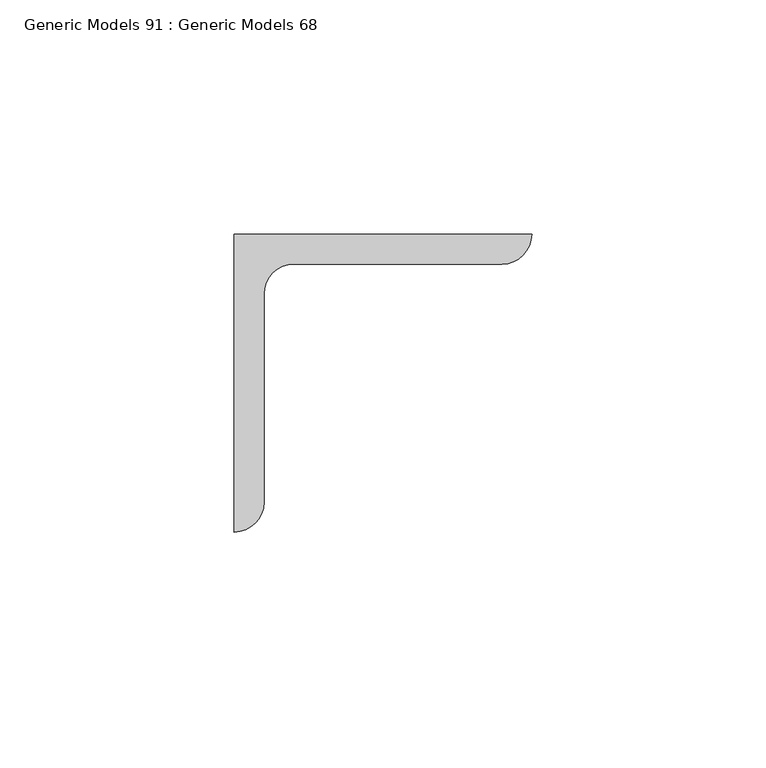
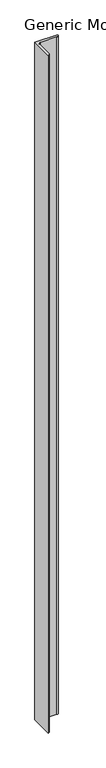
"""IFC4 building model written with IfcOpenShell, lengths in millimetres: proxy geometry, Generic Models 91 : Generic Models 68."""

from ifc_helpers import new_model, si_unit, point, frame, frame_2d, origin, place, context, project, spatial, polyline, circle_curve, trimmed, segment, composite_curve, outline, extrude, source, transform, mapped, element, save


def generic_models_91_generic_models_68_f7824550(model_context):
    return source(origin(), model_context, "Body", "SweptSolid", [
        extrude(outline(composite_curve([segment(polyline([(20530.4116945, 19715.2264581), (20593.9116945, 19715.2264581)]), True, "CONTINUOUS"), segment(trimmed(circle_curve(frame_2d((20587.5616945, 19715.2264581)), 6.35), [point((20593.9116945, 19715.2264581))], [point((20587.5616945, 19708.8764581))], False, "CARTESIAN"), True, "CONTINUOUS"), segment(polyline([(20587.5616945, 19708.8764581), (20543.1116945, 19708.8764581)]), True, "CONTINUOUS"), segment(trimmed(circle_curve(frame_2d((20543.1116945, 19702.5264581)), 6.35), [point((20543.1116945, 19708.8764581))], [point((20536.7616945, 19702.5264581))], True, "CARTESIAN"), True, "CONTINUOUS"), segment(polyline([(20536.7616945, 19702.5264581), (20536.7616945, 19658.0764581)]), True, "CONTINUOUS"), segment(trimmed(circle_curve(frame_2d((20530.4116945, 19658.0764581)), 6.35), [point((20536.7616945, 19658.0764581))], [point((20530.4116945, 19651.7264581))], False, "CARTESIAN"), True, "CONTINUOUS"), segment(polyline([(20530.4116945, 19651.7264581), (20530.4116945, 19715.2264581)]), True, "CONTINUOUS")], self_intersect=False)), frame((0.0, 0.0, 265402.3336948), z_axis=(0.0, 0.0, 1.0), x_axis=(1.0, 0.0, 0.0)), (0.0, 0.0, 1.0), 1984.375),
    ])


if __name__ == "__main__":
    model = new_model("IFC4")
    model_context = context("Model", 3, world=origin())
    ifc_project = project(units=[si_unit("LENGTHUNIT", "METRE", prefix="MILLI")], contexts=[model_context])
    site = spatial("IfcSite", under=ifc_project)
    building = spatial("IfcBuilding", under=site)
    placement = place(None, origin())
    generic_models_91_generic_models_68_shape = generic_models_91_generic_models_68_f7824550(model_context)
    element("IfcBuildingElementProxy", 1, Name="Generic Models 91 : Generic Models 68", ObjectType="Generic Models 91 : Generic Models 68", at=placement, inside=building, context=model_context, shape_type="MappedRepresentation", body=[
        mapped(generic_models_91_generic_models_68_shape, transform((0.0, 0.0, 0.0), x_axis=(1.0, 0.0, 0.0), y_axis=(0.0, 1.0, 0.0), z_axis=(0.0, 0.0, 1.0))),
    ])
    save(model, "model.ifc")

# Revit data of these elements
# Element 1 (IfcBuildingElementProxy, "Generic Models 91 : Generic Models 68")
#   Materials on its faces: "INTERMITTENT FENCE POST:  (2) BACK/BACK GALV. ANGLES (L2 1/2 X 2 1/2 X 1/4\") - NO FOOTING"
# Materials
#   "INTERMITTENT FENCE POST:  (2) BACK/BACK GALV. ANGLES (L2 1/2 X 2 1/2 X 1/4\") - NO FOOTING": class "Unassigned", colour RGB 211 211 211, transparency 0, Cost = 0
